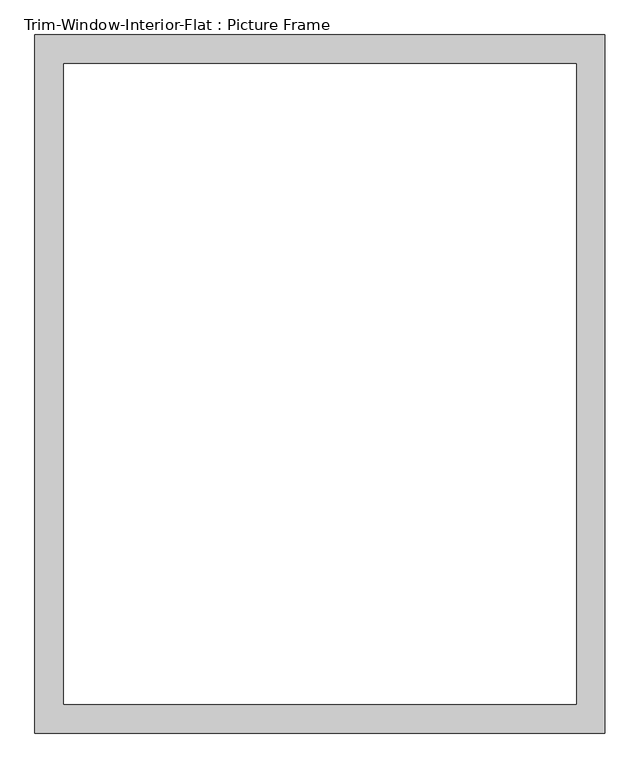
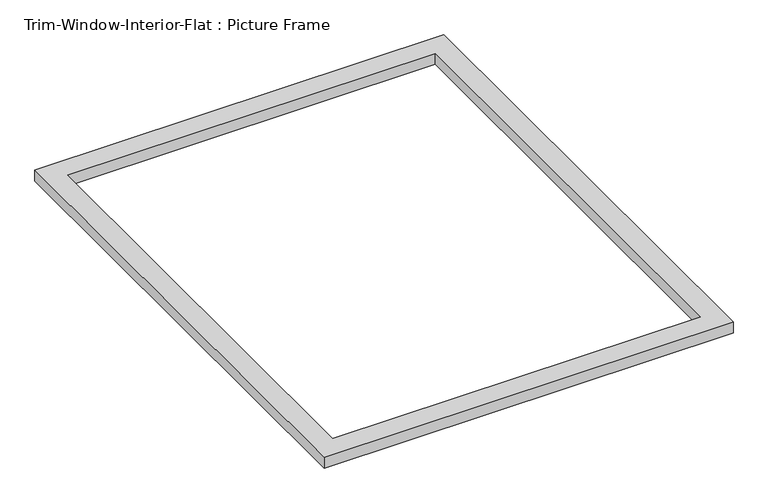
"""IFC4 building model written with IfcOpenShell, lengths in millimetres: proxy geometry, Trim-Window-Interior-Flat : Picture Frame."""

from ifc_helpers import new_model, si_unit, origin, origin_with_axes, place, context, project, spatial, polyline, outline, extrude, source, transform, mapped, element, save


def trim_window_interior_flat_picture_frame_7cb3e35f(model_context):
    return source(origin(), model_context, "Body", "SweptSolid", [
        extrude(outline(polyline([(565.15, -44.45), (-565.15, -44.45), (-565.15, 1339.85), (565.15, 1339.85), (565.15, -44.45)]), holes=[polyline([(508.0, 12.7), (508.0, 1282.7), (-508.0, 1282.7), (-508.0, 12.7), (508.0, 12.7)])]), origin_with_axes(), (0.0, 0.0, 1.0), 31.75),
    ])


if __name__ == "__main__":
    model = new_model("IFC4")
    model_context = context("Model", 3, world=origin())
    ifc_project = project(units=[si_unit("LENGTHUNIT", "METRE", prefix="MILLI")], contexts=[model_context])
    site = spatial("IfcSite", under=ifc_project)
    building = spatial("IfcBuilding", under=site)
    placement = place(None, origin())
    trim_window_interior_flat_picture_frame_shape = trim_window_interior_flat_picture_frame_7cb3e35f(model_context)
    element("IfcBuildingElementProxy", 1, Name="Trim-Window-Interior-Flat : Picture Frame", ObjectType="Trim-Window-Interior-Flat : Picture Frame", at=placement, inside=building, context=model_context, shape_type="MappedRepresentation", body=[
        mapped(trim_window_interior_flat_picture_frame_shape, transform((0.0, 0.0, 0.0), x_axis=(1.0, 0.0, 0.0), y_axis=(0.0, 1.0, 0.0), z_axis=(0.0, 0.0, 1.0))),
    ])
    save(model, "model.ifc")

# Revit data of these elements
# Type "Trim-Window-Interior-Flat : Picture Frame"
#   Trim Thickness_Picture Frame = 0' - 1 1/4"
#   Trim Width = 0' - 2 1/4"
#   Trim Thickness_with Sill = 0' - 0 3/4"
#   Sill Thickness = 0' - 1 1/4"
#   Opening Width [instance default] = 2' - 0"
#   Opening Height [instance default] = 3' - 0"
#   Default Elevation = 4' - 0"
#   Sill = no
#   Picture Frame = yes
#   Trim Material [instance default] = none
# Element 1 (IfcBuildingElementProxy, "Trim-Window-Interior-Flat : Picture Frame")
#   Opening Width = 3' - 5"
#   Opening Height = 4' - 3"
#   Trim Material = Wood - Stained
#   Materials on its faces: "Wood - Stained"
# Materials
#   "Wood - Stained": class "Wood", colour RGB 224 178 126, transparency 0, Cost = 0
